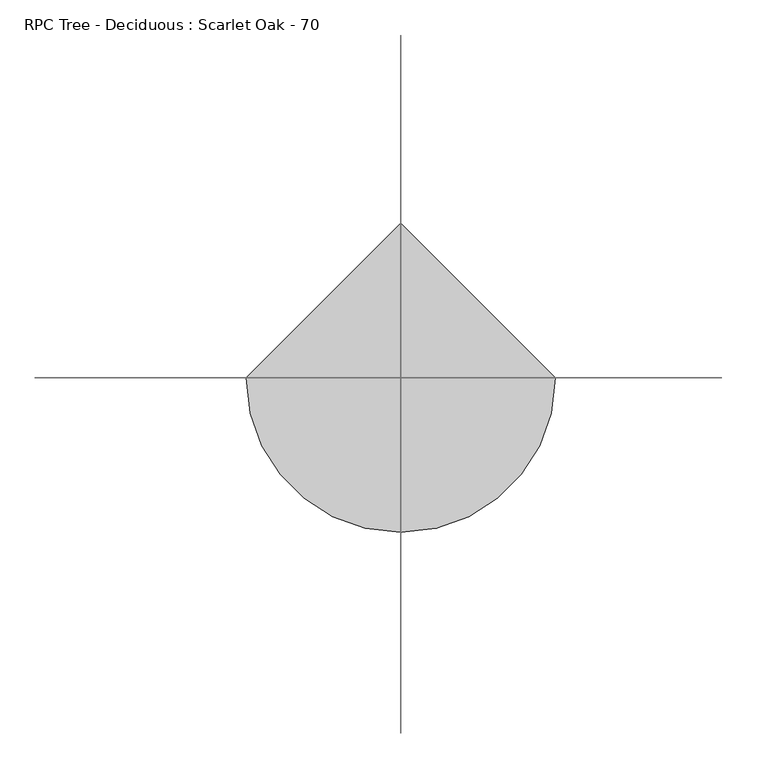
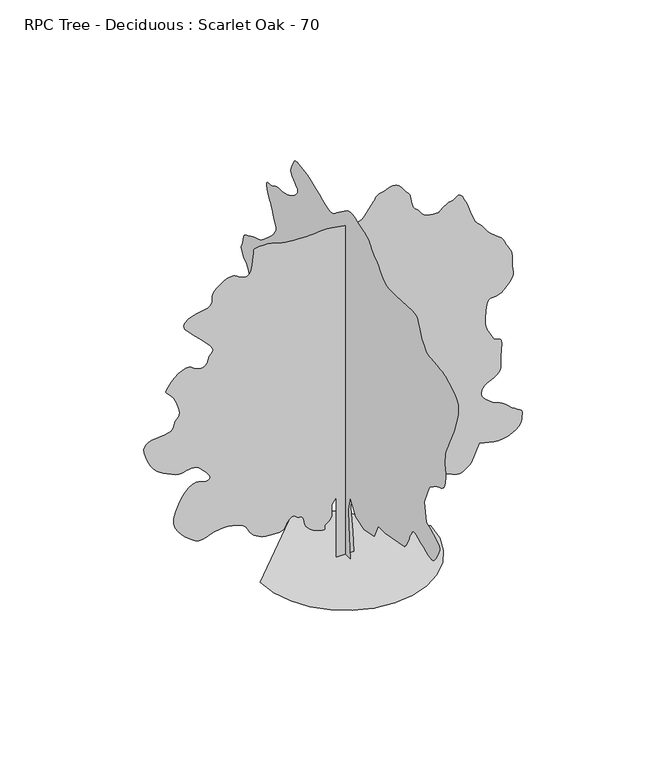
"""IFC4 building model written with IfcOpenShell, lengths in millimetres: geographic element geometry, RPC Tree - Deciduous : Scarlet Oak - 70."""

from ifc_helpers import new_model, si_unit, origin, place, context, project, spatial, triangles, source, transform, mapped, element, save


def rpc_tree_deciduous_scarlet_oak_70_be676745(model_context):
    return source(origin(), model_context, "Body", "Tessellation", [
        triangles([(0.0294444, 522.318082, 0.0), (0.0294444, -501.0802431, 0.0), (0.0294444, -336.0164085, 1947.7549484), (0.0294444, -303.0027805, 2872.1116081), (0.0294444, -501.0802431, 3730.4458443), (0.0294444, -1029.2870281, 2872.1116081), (0.0294444, -1887.6171947, 2608.0102867), (0.0294444, -2878.0002022, 2839.1005417), (0.0294444, -3274.1542191, 3664.4196419), (0.0294444, -3967.424984, 3664.4196419), (0.0294444, -5882.1647964, 4027.5625923), (0.0294444, -5952.6157288, 4112.5481026), (0.0294444, -6021.3603699, 4198.1097404), (0.0294444, -6086.605806, 4284.8236336), (0.0294444, -6146.6457458, 4373.2824783), (0.0294444, -6199.7721542, 4464.0458336), (0.0294444, -6244.2363007, 4557.7110466), (0.0294444, -6278.3313126, 4654.7897141), (0.0294444, -6311.444989, 4754.8129692), (0.0294444, -6353.2209274, 4856.5430969), (0.0294444, -6402.2080536, 4959.7240082), (0.0294444, -6456.956456, 5064.0571747), (0.0294444, -6516.0569183, 5169.2431961), (0.0294444, -6578.0170898, 5275.0274368), (0.0294444, -6641.4701935, 5381.0674759), (0.0294444, -6671.6817215, 5415.3328262), (0.0294444, -6713.4576599, 5442.9840454), (0.0294444, -6778.3193985, 5457.3221237), (0.0294444, -6877.8301849, 5451.7317673), (0.0294444, -7023.555011, 5419.6000076), (0.0294444, -7227.0152664, 5354.2266724), (0.0294444, -7499.7747803, 5249.0400696), (0.0294444, -7787.768248, 5125.2487885), (0.0294444, -8033.0038605, 5014.7706482), (0.0294444, -8241.2859146, 4926.7812515), (0.0294444, -8418.3751053, 4870.5820656), (0.0294444, -8570.0739853, 4855.3908417), (0.0294444, -8702.1008102, 4890.4247498), (0.0294444, -8820.3023163, 4984.9428177), (0.0294444, -8939.5706177, 5133.8255905), (0.0294444, -9062.8503021, 5315.0534821), (0.0294444, -9178.0641998, 5512.4542236), (0.0294444, -9273.0525879, 5709.8549652), (0.0294444, -9335.6946945, 5891.0828568), (0.0294444, -9353.9156754, 6040.0080688), (0.0294444, -9315.5110428, 6140.3728729), (0.0294444, -9221.6754913, 6215.9450043), (0.0294444, -9086.2343399, 6300.1369583), (0.0294444, -8916.1865799, 6391.5831207), (0.0294444, -8718.3591202, 6488.7893967), (0.0294444, -8499.7928101, 6590.3488953), (0.0294444, -8267.3587418, 6694.7675217), (0.0294444, -8028.011142, 6800.6366409), (0.0294444, -7829.9278839, 7923.0809189), (0.0294444, -8325.0935898, 9078.5103928), (0.0294444, -8340.7118225, 9100.5718369), (0.0294444, -8364.9492966, 9127.4981003), (0.0294444, -8406.5548965, 9164.2813202), (0.0294444, -8474.1042618, 9215.7863159), (0.0294444, -8576.3038376, 9286.8779068), (0.0294444, -8721.8583252, 9382.5488113), (0.0294444, -8919.3439453, 9507.7057068), (0.0294444, -9133.6000534, 9621.0854141), (0.0294444, -9323.5762482, 9695.164032), (0.0294444, -9489.3138062, 9755.4161682), (0.0294444, -9630.8144714, 9827.2338776), (0.0294444, -9748.034642, 9936.0039825), (0.0294444, -9841.0167572, 10107.1191193), (0.0294444, -9909.7183777, 10366.0102936), (0.0294444, -9949.4892059, 10620.2924469), (0.0294444, -9960.9245544, 10783.3429596), (0.0294444, -9952.1774139, 10889.2120789), (0.0294444, -9931.2682251, 10971.9953979), (0.0294444, -9906.3476532, 11065.7454895), (0.0294444, -9885.4803223, 11204.5149261), (0.0294444, -9876.7331818, 11422.4411591), (0.0294444, -9879.8050873, 11662.8555542), (0.0294444, -9893.2903107, 11862.2608246), (0.0294444, -9923.5012573, 12044.3857544), (0.0294444, -9976.7991669, 12232.825415), (0.0294444, -10059.582486, 12451.3051025), (0.0294444, -10178.1682709, 12723.5105804), (0.0294444, -10338.8712524, 13073.0787781), (0.0294444, -10491.4654266, 13389.0653046), (0.0294444, -10593.1964264, 13579.7234344), (0.0294444, -10661.9829254, 13697.6267029), (0.0294444, -10715.7924316, 13795.303299), (0.0294444, -10772.5040863, 13925.3244324), (0.0294444, -10849.9528473, 14140.2636383), (0.0294444, -10966.1492432, 14492.6060852), (0.0294444, -11091.3485779, 14900.2091125), (0.0294444, -11175.5829712, 15251.2283844), (0.0294444, -11206.0938995, 15553.7308502), (0.0294444, -11170.1635345, 15815.8218292), (0.0294444, -11055.1635773, 16045.5682709), (0.0294444, -10848.332016, 16251.0336365), (0.0294444, -10536.9545105, 16440.369754), (0.0294444, -10234.8369049, 16595.9939758), (0.0294444, -10036.1129883, 16703.1432495), (0.0294444, -9898.5806854, 16773.8505615), (0.0294444, -9780.0809418, 16820.3640015), (0.0294444, -9638.4953979, 16854.7142303), (0.0294444, -9431.664418, 16889.0656219), (0.0294444, -9117.4277847, 16935.5778992), (0.0294444, -8780.3611496, 16972.2338013), (0.0294444, -8518.9526871, 16986.4003784), (0.0294444, -8311.8228882, 17003.9807007), (0.0294444, -8137.6358459, 17051.0487579), (0.0294444, -7974.9701935, 17153.5471527), (0.0294444, -7802.4900238, 17337.5056915), (0.0294444, -7598.8164093, 17628.8274445), (0.0294444, -7420.9592422, 17949.1230103), (0.0294444, -7315.8580994, 18206.5212524), (0.0294444, -7247.1564789, 18406.6950806), (0.0294444, -7178.4118378, 18555.4929749), (0.0294444, -7073.3106949, 18658.6738861), (0.0294444, -6895.4541092, 18721.9990906), (0.0294444, -6608.4419769, 18751.2717224), (0.0294444, -5023.817189, 18652.2300934), (0.0294444, -4731.7274597, 18657.3507111), (0.0294444, -4493.916394, 18656.6681946), (0.0294444, -4291.8644829, 18668.701181), (0.0294444, -4107.1713959, 18711.8857544), (0.0294444, -3921.3179146, 18804.7824097), (0.0294444, -3715.830748, 18965.7842102), (0.0294444, -3472.2290474, 19213.451651), (0.0294444, -3237.4861084, 19463.5956848), (0.0294444, -3061.6392838, 19634.0271423), (0.0294444, -2930.8408722, 19746.1691345), (0.0294444, -2831.2231155, 19821.3575684), (0.0294444, -2748.9345337, 19880.9283508), (0.0294444, -2670.1064964, 19946.2592468), (0.0294444, -2580.8878143, 20038.7722046), (0.0294444, -2495.2282173, 20148.0120483), (0.0294444, -2425.156477, 20249.7407227), (0.0294444, -2353.9368416, 20344.5581909), (0.0294444, -2264.8121944, 20432.9760498), (0.0294444, -2141.0377728, 20515.6733276), (0.0294444, -1965.8648895, 20593.166272), (0.0294444, -1722.5534328, 20666.006012), (0.0294444, -1449.4057159, 20746.2732056), (0.0294444, -1194.7349236, 20835.2003357), (0.0294444, -956.808676, 20917.2162598), (0.0294444, -733.9029505, 20976.701001), (0.0294444, -524.2767197, 20998.0810913), (0.0294444, -326.1984395, 20965.7342285), (0.0294444, -137.9389459, 20864.08927), (0.0294444, 852.4457148, 20137.8126709), (0.0294444, 959.6634436, 20040.2209534), (0.0294444, 1063.4204098, 19951.2938232), (0.0294444, 1176.4115507, 19879.6470337), (0.0294444, 1311.3532413, 19834.0312134), (0.0294444, 1480.9402737, 19823.0644409), (0.0294444, 1697.8805202, 19855.4089783), (0.0294444, 1974.8814903, 19939.7294128), (0.0294444, 2289.2248032, 20064.9287476), (0.0294444, 2605.876696, 20205.7457336), (0.0294444, 2919.0633934, 20349.4671936), (0.0294444, 3223.0119919, 20483.3287903), (0.0294444, 3511.9481346, 20594.701062), (0.0294444, 3780.0904884, 20670.8289734), (0.0294444, 4021.6737076, 20699.0342285), (0.0294444, 4241.4047722, 20714.4402649), (0.0294444, 4445.5263245, 20749.4730103), (0.0294444, 4630.6374092, 20787.3660461), (0.0294444, 4793.1751625, 20811.432019), (0.0294444, 4929.7682785, 20804.9045105), (0.0294444, 5036.8751129, 20751.0101257), (0.0294444, 5111.0816299, 20632.9777954), (0.0294444, 5177.3938614, 20484.6938232), (0.0294444, 5253.52061, 20347.9300781), (0.0294444, 5325.0389191, 20218.0798645), (0.0294444, 5377.5252502, 20090.5318359), (0.0294444, 5396.4717682, 19960.7234802), (0.0294444, 5367.497374, 19823.9597351), (0.0294444, 5276.1796921, 19675.6315796), (0.0294444, 5136.42892, 19539.7212708), (0.0294444, 4986.82061, 19433.2556763), (0.0294444, 4849.971405, 19341.2543152), (0.0294444, 4748.3267372, 19248.6564789), (0.0294444, 4704.459938, 19140.4828491), (0.0294444, 4740.8164398, 19001.7134125), (0.0294444, 4880.0125946, 18817.2851349), (0.0294444, 5072.2072586, 18633.5393738), (0.0294444, 5253.4351501, 18499.5068573), (0.0294444, 5424.8485245, 18404.0917511), (0.0294444, 5587.5996368, 18336.4575073), (0.0294444, 5742.8401611, 18285.5071289), (0.0294444, 5891.7659546, 18240.4029053), (0.0294444, 6035.4420685, 18190.0490021), (0.0294444, 6178.9484253, 18151.260672), (0.0294444, 6326.5080231, 18138.4591278), (0.0294444, 6478.0790039, 18137.221994), (0.0294444, 6633.7038071, 18133.0827118), (0.0294444, 6793.3824326, 18111.6189056), (0.0294444, 6957.1148804, 18058.3640167), (0.0294444, 7124.8587112, 17958.9805481), (0.0294444, 7298.2347565, 17870.6917511), (0.0294444, 7468.6667953, 17839.0297302), (0.0294444, 7621.2191116, 17831.6046021), (0.0294444, 7740.8716919, 17816.1148499), (0.0294444, 7812.5603394, 17760.2147736), (0.0294444, 7821.3080612, 17631.5156525), (0.0294444, 7752.136702, 17397.7589905), (0.0294444, 7649.8946869, 17151.7542389), (0.0294444, 7565.0202164, 16986.0166809), (0.0294444, 7490.5148804, 16867.6018158), (0.0294444, 7419.5087494, 16763.6523468), (0.0294444, 7345.0034134, 16641.2260986), (0.0294444, 7260.0859222, 16467.4239166), (0.0294444, 7157.8863464, 16209.3001373), (0.0294444, 7049.8836365, 15955.4016815), (0.0294444, 6956.9439606, 15795.0405396), (0.0294444, 6885.8953903, 15696.4686493), (0.0294444, 6843.735173, 15627.9367859), (0.0294444, 6837.3774216, 15557.6992126), (0.0294444, 6873.7763626, 15453.9206635), (0.0294444, 6959.8030884, 15284.9402802), (0.0294444, 7112.9530426, 15060.953952), (0.0294444, 7327.8492279, 14823.1428864), (0.0294444, 7577.4374817, 14585.886438), (0.0294444, 7834.4938843, 14363.6511658), (0.0294444, 8071.9636917, 14170.8594452), (0.0294444, 8262.6218216, 14021.9766724), (0.0294444, 8379.3728348, 13931.3833649), (0.0294444, 8483.0229034, 13874.7158936), (0.0294444, 8638.6477066, 13817.4496216), (0.0294444, 8825.4659546, 13759.0310944), (0.0294444, 9022.6957764, 13698.8638367), (0.0294444, 9209.513443, 13636.3920685), (0.0294444, 9365.1382462, 13571.0611725), (0.0294444, 9468.7888962, 13502.2316528), (0.0294444, 9555.5835983, 13445.0514221), (0.0294444, 9666.1041779, 13404.641098), (0.0294444, 9787.5490906, 13365.3830292), (0.0294444, 9907.285968, 13311.6584015), (0.0294444, 10012.60047, 13227.9356049), (0.0294444, 10090.7329102, 13098.5539673), (0.0294444, 10129.0526642, 12907.9807159), (0.0294444, 10160.4170288, 12716.555191), (0.0294444, 10214.3114136, 12581.1564789), (0.0294444, 10272.8148193, 12480.9625946), (0.0294444, 10318.0899628, 12395.1922485), (0.0294444, 10332.1286407, 12303.1060089), (0.0294444, 10297.0947327, 12183.8377075), (0.0294444, 10195.0660767, 12016.6490753), (0.0294444, 10068.4156677, 11860.0423553), (0.0294444, 9966.0033142, 11766.420163), (0.0294444, 9879.7632294, 11705.6971252), (0.0294444, 9801.5877686, 11647.8343781), (0.0294444, 9723.4553284, 11562.831427), (0.0294444, 9637.2152435, 11420.6912659), (0.0294444, 9534.8023087, 11191.3296844), (0.0294444, 9423.1724945, 10961.5832428), (0.0294444, 9320.7595596, 10816.7548737), (0.0294444, 9236.8239853, 10724.4546936), (0.0294444, 9180.6245087, 10652.339328), (0.0294444, 9161.3797531, 10568.1479553), (0.0294444, 9188.3060165, 10439.4488342), (0.0294444, 9270.7056381, 10233.9834686), (0.0294444, 9380.1588409, 10009.2297455), (0.0294444, 9483.211853, 9834.7438843), (0.0294444, 9581.6988647, 9696.0599075), (0.0294444, 9677.2412888, 9578.7118378), (0.0294444, 9771.6744781, 9468.3191574), (0.0294444, 9866.6628662, 9350.4164703), (0.0294444, 9963.9546021, 9210.5802383), (0.0294444, 10076.865152, 9072.6648193), (0.0294444, 10208.2513184, 8960.1385483), (0.0294444, 10344.2476685, 8858.0244324), (0.0294444, 10471.0259766, 8751.2588562), (0.0294444, 10574.6766266, 8624.9072662), (0.0294444, 10641.3725555, 8463.8630264), (0.0294444, 10657.247168, 8253.1915833), (0.0294444, 10670.6033295, 8087.7522629), (0.0294444, 10719.8038147, 8033.1747803), (0.0294444, 10775.9178314, 8030.5714508), (0.0294444, 10810.0983032, 8021.0557526), (0.0294444, 10793.4132751, 7945.6969803), (0.0294444, 10697.1028748, 7745.6080307), (0.0294444, 10492.1909637, 7361.8587799), (0.0294444, 10277.935437, 6931.4263321), (0.0294444, 10148.5968201, 6614.8003098), (0.0294444, 10067.7331512, 6388.2118149), (0.0294444, 9999.0315308, 6228.064032), (0.0294444, 9906.0488342, 6110.6305023), (0.0294444, 9752.4297226, 6012.2713898), (0.0294444, 9501.8171127, 5909.3038376), (0.0294444, 9212.4580307, 5825.7519608), (0.0294444, 8957.7915985, 5790.718634), (0.0294444, 8723.906456, 5788.0298447), (0.0294444, 8496.9767029, 5801.5144867), (0.0294444, 8263.0915604, 5814.9561081), (0.0294444, 8008.4251282, 5812.2679001), (0.0294444, 7719.1084854, 5777.233992), (0.0294444, 7430.5609818, 5745.8702087), (0.0294444, 7181.2709656, 5752.6122391), (0.0294444, 6962.022139, 5778.9838852), (0.0294444, 6763.5546021, 5806.5072052), (0.0294444, 6576.6514755, 5816.7054199), (0.0294444, 6392.0522781, 5791.1023315), (0.0294444, 6200.4976913, 5711.2205795), (0.0294444, 6017.1786484, 5626.3030884), (0.0294444, 5865.5652283, 5581.838942), (0.0294444, 5749.198494, 5553.5476456), (0.0294444, 5671.5357925, 5517.1911438), (0.0294444, 5636.0321457, 5448.4465027), (0.0294444, 5646.1454819, 5323.1611267), (0.0294444, 5705.3319855, 5116.970224), (0.0294444, 5800.7889496, 4897.9347565), (0.0294444, 5915.3209122, 4742.9500305), (0.0294444, 6045.7687637, 4641.4335526), (0.0294444, 6188.8908417, 4582.6313278), (0.0294444, 6341.5286179, 4555.8759842), (0.0294444, 6500.5247269, 4550.4568382), (0.0294444, 6662.6782013, 4555.748085), (0.0294444, 7289.956192, 3862.4988304), (0.0294444, 7339.1148193, 3784.4387695), (0.0294444, 7386.2671738, 3704.9410057), (0.0294444, 7429.4087265, 3622.554174), (0.0294444, 7466.4477448, 3535.8318512), (0.0294444, 7495.422139, 3443.3401131), (0.0294444, 7514.283197, 3343.6284668), (0.0294444, 7521.0252274, 3235.2545586), (0.0294444, 7519.8729721, 3122.2591301), (0.0294444, 7511.8083481, 3010.4200264), (0.0294444, 7489.8323639, 2900.8938629), (0.0294444, 7447.1175293, 2794.828244), (0.0294444, 7376.6660156, 2693.3841454), (0.0294444, 7271.5648727, 2597.7135315), (0.0294444, 7124.8587112, 2508.9727272), (0.0294444, 6984.9370193, 2433.6097401), (0.0294444, 6886.5779068, 2374.9954399), (0.0294444, 6802.6423325, 2329.6650673), (0.0294444, 6705.9900925, 2294.1490665), (0.0294444, 6569.5251663, 2264.9870384), (0.0294444, 6366.0649109, 2238.7097179), (0.0294444, 6068.470285, 2211.8561245), (0.0294444, 5729.9537384, 2215.7051628), (0.0294444, 5418.0210342, 2274.9936951), (0.0294444, 5126.8702011, 2376.4421539), (0.0294444, 4850.7396721, 2506.7580368), (0.0294444, 4583.869043, 2652.6706421), (0.0294444, 4320.4118683, 2800.8918274), (0.0294444, 4054.684774, 2938.1378105), (0.0294444, 3817.7230751, 3062.9705978), (0.0294444, 3634.4679817, 3180.8732849), (0.0294444, 3489.9038406, 3288.9614548), (0.0294444, 3369.0184868, 3384.3419701), (0.0294444, 3256.7953949, 3464.1301231), (0.0294444, 3138.2183304, 3525.4412064), (0.0294444, 2998.2754189, 3565.3820824), (0.0294444, 2844.3746384, 3599.0675262), (0.0294444, 2692.7867981, 3640.8391045), (0.0294444, 2541.7747948, 3686.6560753), (0.0294444, 2389.6106815, 3732.4686859), (0.0294444, 2234.5534309, 3774.2402641), (0.0294444, 2074.8790203, 3807.9254173), (0.0294444, 1908.8551426, 3829.4834038), (0.0294444, 1739.0759708, 3840.744635), (0.0294444, 1569.2927296, 3846.8082184), (0.0294444, 1399.5135578, 3848.5406708), (0.0294444, 1229.7345314, 3846.8082184), (0.0294444, 1059.9554323, 3842.4770874), (0.0294444, 890.1720457, 3836.4132133), (0.0294444, 720.3929466, 3829.4834038), (0.0294444, 390.2661495, 3334.2918274), (0.0294444, 324.2397655, 2574.9992203), (478.6859705, 0.0010255, 0.0157241), (-511.6970369, 0.0010255, 0.0157241), (-511.6970369, 0.0008118, 3631.4213654), (-775.8025732, 0.0008118, 3268.2824844), (-775.8025732, 0.0008546, 2872.1284676), (-769.7388445, 0.0008546, 2780.2131477), (-769.7388445, 0.0008546, 2688.5835663), (-781.8662292, 0.0008546, 2597.534182), (-812.1804399, 0.0008973, 2507.3513145), (-866.753635, 0.0008973, 2418.3246265), (-951.6453283, 0.0008973, 2330.7360775), (-1072.9148884, 0.0008973, 2244.884341), (-1167.9112701, 0.0008973, 2155.7595486), (-1194.188736, 0.0008973, 2065.4784313), (-1188.1250072, 0.0008973, 1985.0204063), (-1186.1023836, 0.0008973, 1925.3435257), (-1224.5072342, 0.0008973, 1897.4318573), (-1339.7129929, 0.0008973, 1912.2560978), (-1568.1063194, 0.0008973, 1980.7830196), (-1828.6488464, 0.0008973, 2087.5227253), (-2023.3568745, 0.0008973, 2208.1181259), (-2163.2015362, 0.0008973, 2340.2690712), (-2259.162394, 0.0008973, 2481.6540459), (-2322.2059296, 0.0008546, 2629.9691208), (-2363.303421, 0.0008546, 2782.9057159), (-2393.4297798, 0.0008546, 2938.1549606), (-2401.1278564, 0.0008546, 2980.4044167), (-2412.5809364, 0.0008546, 3021.5019081), (-2431.540099, 0.0008546, 3060.2948891), (-2461.7648529, 0.0008546, 3095.6145355), (-2506.9969757, 0.0008546, 3126.3170219), (-2571.0049873, 0.0008546, 3151.2460236), (-2657.5311012, 0.0008546, 3169.2452156), (-2744.0572151, 0.0008546, 3198.8852669), (-2812.101899, 0.0008546, 3248.7429794), (-2871.4883904, 0.0008118, 3302.6420151), (-2932.027137, 0.0008118, 3344.4135933), (-3003.5413765, 0.0008118, 3357.8895149), (-3095.8406845, 0.0008118, 3326.8969299), (-3218.74888, 0.0008546, 3235.2673485), (-3326.8329803, 0.0008546, 3107.0679062), (-3388.1440636, 0.0008546, 2981.7528809), (-3432.7064598, 0.0008546, 2866.2570236), (-3490.548278, 0.0008546, 2767.5054932), (-3591.7066383, 0.0008546, 2692.4368195), (-3766.2009293, 0.0008546, 2647.9683128), (-4044.0679802, 0.0008546, 2641.0382126), (-4351.0931351, 0.0008546, 2661.4442345), (-4600.3828606, 0.0008546, 2695.1293877), (-4802.8614899, 0.0008546, 2743.2549385), (-4969.5809647, 0.0008546, 2806.9684914), (-5111.4653275, 0.0008546, 2887.4307312), (-5239.4389114, 0.0008546, 2985.7982735), (-5364.5958069, 0.0008546, 3103.2187225), (-5470.7213058, 0.0008546, 3231.9942924), (-5546.8904938, 0.0008118, 3361.3544197), (-5611.4534134, 0.0008118, 3487.8214096), (-5682.9717224, 0.0008118, 3607.9390778), (-5779.8797607, 0.0008118, 3718.2375778), (-5920.6973282, 0.0008118, 3815.2566559), (-6123.8587646, 0.0008118, 3895.5267563), (-6328.1294357, 0.0008118, 3956.5436714), (-6476.3296921, 0.0007691, 3999.6637138), (-6593.3789429, 0.0007691, 4027.191394), (-6704.0698608, 0.0007691, 4041.4352921), (-6833.1951187, 0.0007691, 4044.7080574), (-7005.6758698, 0.0007691, 4039.3188515), (-7246.3030426, 0.0007691, 4027.5753822), (-7510.8694519, 0.0007691, 3985.9020538), (-7746.0347488, 0.0008118, 3908.4224808), (-7962.6808273, 0.0008118, 3824.0128075), (-8171.8157364, 0.0008118, 3761.549469), (-8384.4504318, 0.0008118, 3749.9045403), (-8611.4656448, 0.0008118, 3817.9492241), (-8863.9130264, 0.0007691, 3994.5643158), (-9128.0527176, 0.0007691, 4230.7539688), (-9371.9232971, 0.0007691, 4465.1980888), (-9579.4373749, 0.0007264, 4708.3431313), (-9734.3790802, 0.0007264, 4970.5198608), (-9820.619165, 0.0007264, 5262.1404327), (-9821.9853607, 0.0006837, 5593.6167114), (-9722.2606339, 0.0006837, 5975.3172501), (-9555.3702393, 0.0006409, 6360.304216), (-9369.4054276, 0.0006409, 6690.4573196), (-9169.6152969, 0.0005982, 6959.3763702), (-8961.1629044, 0.0005982, 7160.703035), (-8749.2107254, 0.0005982, 7288.1214203), (-8539.0084396, 0.0005982, 7335.3167953), (-8335.719104, 0.0005982, 7295.8453674), (-8143.9935974, 0.0005982, 7229.4476761), (-7974.2446564, 0.0005982, 7201.1133591), (-7840.2545792, 0.0005982, 7212.6771881), (-7755.934726, 0.0005982, 7265.8041779), (-7735.1534363, 0.0005982, 7362.2430588), (-7791.7366104, 0.0005982, 7503.7431427), (-7939.5525879, 0.0005555, 7692.0118835), (-8111.9472977, 0.0005555, 7880.8358231), (-8243.3340454, 0.0005555, 8026.34729), (-8349.2886246, 0.0005555, 8133.7523621), (-8445.4286865, 0.0005555, 8208.2576981), (-8547.372464, 0.0005555, 8255.026355), (-8670.6515671, 0.0005127, 8279.3068497), (-8830.9278305, 0.0005127, 8286.2197998), (-8995.3003555, 0.0005555, 8270.7294662), (-9131.4240234, 0.0005555, 8235.0130417), (-9255.3862244, 0.0005555, 8195.2858154), (-9383.4022476, 0.0005555, 8167.6340149), (-9531.6019226, 0.0005555, 8168.3171127), (-9716.20112, 0.0005555, 8213.4637756), (-9953.3715271, 0.0005127, 8319.2480164), (-10205.0515137, 0.0005127, 8445.8129654), (-10426.6903107, 0.0005127, 8555.6080078), (-10624.6875275, 0.0005127, 8668.3476379), (-10805.3183624, 0.0005127, 8803.5748489), (-10975.0254456, 0.0005127, 8980.919838), (-11140.0804871, 0.00047, 9220.0965179), (-11306.8854218, 0.00047, 9540.7339233), (-11444.8014221, 0.0004273, 9873.4473358), (-11520.9281708, 0.0004273, 10140.9158936), (-11538.1678162, 0.0004273, 10350.6484406), (-11499.3783234, 0.0003846, 10510.1131256), (-11407.4630035, 0.0003846, 10626.8641388), (-11265.3228424, 0.0003846, 10708.3673035), (-11075.7739471, 0.0003846, 10762.1768097), (-10852.0015594, 0.0003846, 10793.0714355), (-10615.5566895, 0.0003846, 10811.2924164), (-10381.9267639, 0.0003846, 10832.3295044), (-10166.8178009, 0.0003846, 10871.8863922), (-9985.8032684, 0.0003846, 10945.5388733), (-9854.4159393, 0.0003846, 11068.8185577), (-9788.2746277, 0.0003418, 11257.3861176), (-9739.4148193, 0.0003418, 11439.466864), (-9663.9275665, 0.0003418, 11558.0526489), (-9583.8748947, 0.0003418, 11650.6504852), (-9521.1048889, 0.0003418, 11754.770874), (-9497.6348099, 0.0002991, 11908.0057068), (-9535.356926, 0.0002991, 12147.8654846), (-9656.24664, 0.0002991, 12511.8572205), (-9827.4466553, 0.0002564, 12870.3876617), (-9991.1796844, 0.0002564, 13096.0796997), (-10131.7838928, 0.0002564, 13229.984317), (-10233.7265076, 0.0002136, 13313.0234344), (-10281.3491821, 0.0002136, 13386.2491974), (-10259.1168182, 0.0002136, 13490.7102631), (-10151.4129272, 0.0002136, 13667.329715), (-9977.8235229, 0.0002136, 13887.7302155), (-9777.0508942, 0.0001709, 14088.5016815), (-9562.4110886, 0.0001709, 14258.0808655), (-9347.173645, 0.0001709, 14384.9440521), (-9144.694725, 0.0001709, 14457.4872986), (-8968.160733, 0.0001709, 14464.2287476), (-8830.9278305, 0.0001709, 14393.6074768), (-8696.383136, 0.0001709, 14288.2929749), (-8530.6449966, 0.0001709, 14206.106131), (-8351.0385178, 0.0001709, 14157.9718597), (-8174.8882233, 0.0001709, 14154.8999542), (-8019.5622391, 0.0001709, 14207.8560242), (-7902.3420685, 0.0001709, 14327.7638214), (-7840.5533981, 0.0001709, 14525.6343018), (-7783.9277847, 0.0001709, 14714.2867401), (-7694.9989105, 0.0001282, 14826.1299133), (-7610.12444, 0.0001282, 14901.5741455), (-7565.6602936, 0.0001282, 14981.0727814), (-7598.0054123, 0.0001282, 15105.0349823), (-7743.5168793, 0.0001282, 15313.914093), (-8038.6366562, 8.55e-05, 15648.0785797), (-8408.6884872, 8.55e-05, 16025.5543762), (-8739.4816681, 4.27e-05, 16343.5465942), (-9007.9309799, 4.27e-05, 16611.3139709), (-9190.8663254, 4.27e-05, 16838.0722229), (-9265.2862015, 0.0, 17033.0835754), (-9208.0199295, 0.0, 17205.5637451), (-8995.982872, 0.0, 17364.7307739), (-8713.1954819, 0.0, 17487.3697998), (-8459.894664, 0.0, 17557.437616), (-8237.189653, 0.0, 17595.1585693), (-8046.2321228, -4.27e-05, 17620.7628204), (-7888.1754913, -4.27e-05, 17654.4305328), (-7764.2132904, -4.27e-05, 17716.4325623), (-7675.455336, -4.27e-05, 17826.9107025), (-7631.2045486, -4.27e-05, 17957.6155151), (-7624.4625183, -4.27e-05, 18072.1468964), (-7632.1434448, -4.27e-05, 18178.6136536), (-7631.2045486, -4.27e-05, 18285.0804108), (-7598.4751511, -8.55e-05, 18399.611792), (-7510.8694519, -8.55e-05, 18530.3154419), (-7345.3446716, -8.55e-05, 18685.2583099), (-7142.7378525, -8.55e-05, 18838.5780212), (-6957.4561386, -8.55e-05, 18957.8463226), (-6786.6404022, -0.0001282, 19041.2703003), (-6627.3454742, -0.0001282, 19087.1861023), (-6476.7133896, -0.0001282, 19093.8426727), (-6331.8419998, -0.0001282, 19059.4482605), (-6189.9151978, -8.55e-05, 18982.383197), (-6043.5927338, -8.55e-05, 18888.1633667), (-5892.7042694, -8.55e-05, 18814.724826), (-5744.6755142, -8.55e-05, 18778.7956238), (-5607.0153122, -8.55e-05, 18797.1863617), (-5487.2778534, -8.55e-05, 18886.5843933), (-5392.9725632, -0.0001282, 19063.8014832), (-5331.5675903, -0.0001282, 19345.5214966), (-5294.9122696, -0.0001282, 19648.0239624), (-5268.6266647, -0.0001709, 19881.7817871), (-5251.0027405, -0.0001709, 20054.9433105), (-5240.334787, -0.0001709, 20175.5359497), (-5234.8304718, -0.0001709, 20251.6615356), (-5232.8247803, -0.0001709, 20291.4312012), (-5232.5259613, -0.0001709, 20302.8677124), (-5189.1286102, -0.0001709, 20309.6114868), (-5071.2259232, -0.0001709, 20324.4594177), (-4897.2946793, -0.0001709, 20339.2678162), (-4685.854969, -0.0001709, 20346.0092651), (-4455.3408417, -0.0001709, 20336.5796082), (-4224.242157, -0.0001709, 20302.8677124), (-4011.0569138, -0.0001709, 20236.8554626), (-3815.5766945, -0.0001709, 20163.4157593), (-3619.5200569, -0.0001709, 20110.2050537), (-3414.2250298, -0.0001709, 20073.1212708), (-3191.0249908, -0.0001709, 20048.2018616), (-2941.2658173, -0.0001709, 20031.3889343), (-2656.2765266, -0.0001709, 20018.5873901), (-2327.3992172, -0.0001709, 20005.7858459), (-2009.9792027, -0.0001709, 20003.9510742), (-1748.5705948, -0.0001709, 20019.4408264), (-1518.346566, -0.0001709, 20041.2883301), (-1294.4765099, -0.0001709, 20058.5291382), (-1052.1293839, -0.0001709, 20060.1499695), (-766.4659338, -0.0001709, 20035.2305603), (-412.6608582, -0.0001709, 19972.7576294), (-55.0054861, -0.0001709, 19898.4668152), (233.3518357, -0.0001709, 19847.258313), (463.9598708, -0.0001709, 19822.0412476), (648.37118, -0.0001709, 19825.6666077), (798.1328236, -0.0001709, 19861.1272339), (924.7918802, -0.0001709, 19931.19505), (1039.9038219, -0.0001709, 20038.7722046), (1535.0953983, -0.0002136, 20666.006012), (1609.4000198, -0.0002136, 20762.7442932), (1668.6885521, -0.0002136, 20853.7201355), (1722.1992393, -0.0002136, 20937.1452759), (1779.1791916, -0.0002136, 21011.3523743), (1848.8625835, -0.0002136, 21074.5903748), (1940.492165, -0.0002136, 21125.1151978), (2063.3021107, -0.0002136, 21161.2153198), (2213.831876, -0.0002564, 21202.6081421), (2378.2215511, -0.0002564, 21257.8675598), (2550.1170181, -0.0002564, 21308.4760986), (2723.1733154, -0.0002564, 21336.0), (2891.0278954, -0.0002564, 21321.961322), (3047.3311455, -0.0002564, 21247.8402649), (3185.7378136, -0.0002136, 21095.2007446), (3308.6419395, -0.0002136, 20921.0997437), (3421.15513, -0.0002136, 20785.6591736), (3520.9647354, -0.0002136, 20675.0542969), (3605.7583969, -0.0002136, 20575.4580505), (3673.2269531, -0.0002136, 20472.9596558), (3721.0624054, -0.0001709, 20353.6901917), (3746.9515228, -0.0001709, 20203.8272461), (3764.9504242, -0.0001709, 20048.4995178), (3789.8794258, -0.0001709, 19919.1609009), (3820.5819122, -0.0001709, 19811.4581726), (3855.9015587, -0.0001282, 19721.0776428), (3894.6904701, -0.0001282, 19643.6707397), (3935.7879616, -0.0001282, 19574.970282), (3978.0417778, -0.0001282, 19510.5765381), (4020.7734718, -0.0001282, 19481.6027252), (4065.2419785, -0.0001282, 19448.5745087), (4113.1710297, -0.0001282, 19407.4816681), (4166.3020889, -0.0001282, 19354.2697998), (4226.3585976, -0.0001282, 19284.8845001), (4295.0648689, -0.0001282, 19195.2736908), (4374.1786446, -0.0001282, 19081.424826), (4491.4412544, -8.55e-05, 18973.2081757), (4657.1793938, -8.55e-05, 18899.1301392), (4847.1550072, -8.55e-05, 18852.7027405), (5037.1309113, -8.55e-05, 18827.69729), (5202.8690506, -8.55e-05, 18817.6688324), (5320.1316605, -8.55e-05, 18816.3468201), (5364.5958069, -8.55e-05, 18817.3281555), (5387.3827881, -8.55e-05, 18841.0964722), (5450.0679153, -8.55e-05, 18902.3729645), (5543.9034668, -8.55e-05, 18986.2236603), (5660.2702011, -0.0001282, 19077.5413422), (5790.4622543, -0.0001282, 19161.392038), (5925.9034058, -0.0001282, 19222.7115509), (6057.8453522, -0.0001282, 19246.4798676), (6176.1317368, -0.0001282, 19275.4548431), (6280.5503632, -0.0001282, 19340.7857391), (6377.5008408, -0.0001282, 19410.1698761), (6473.2572052, -0.0001282, 19451.3057373), (6574.2190659, -0.0001282, 19431.7615814), (6686.7453369, -0.0001282, 19319.2358917), (6817.1507492, -0.0001282, 19081.424826), (6939.9606949, -8.55e-05, 18802.0081604), (7031.5777771, -8.55e-05, 18576.3161224), (7101.260733, -8.55e-05, 18389.2845154), (7158.228186, -4.27e-05, 18225.9793671), (7211.7388733, -4.27e-05, 18071.2934601), (7271.0526947, -4.27e-05, 17910.2916595), (7345.3446716, -4.27e-05, 17727.8690735), (7421.6847794, 0.0, 17567.8067505), (7487.0156754, 0.0, 17466.0757507), (7550.6396988, 0.0, 17396.1369965), (7621.7737289, 0.0, 17331.3607178), (7709.6358078, 0.0, 17245.2055115), (7823.4846725, 0.0, 17111.1311371), (7972.5802231, 0.0, 16902.5496826), (8156.1126251, 4.27e-05, 16670.4138519), (8357.567189, 4.27e-05, 16476.3849976), (8562.4779373, 4.27e-05, 16310.0486389), (8756.4224945, 8.55e-05, 16161.0809875), (8924.9343018, 8.55e-05, 16019.025705), (9053.6328415, 8.55e-05, 15873.4717987), (9128.0527176, 8.55e-05, 15714.0919922), (9186.4706635, 8.55e-05, 15557.7840912), (9267.9744095, 0.0001282, 15417.6496216), (9359.335112, 0.0001282, 15277.515152), (9447.1966095, 0.0001282, 15121.207251), (9518.331221, 0.0001282, 14932.5966705), (9559.4240616, 0.0001709, 14695.4262634), (9557.205011, 0.0001709, 14393.6074768), (9552.6820313, 0.0001709, 14103.5228577), (9577.6026031, 0.0002136, 13891.9543762), (9604.8271042, 0.0002136, 13728.3504089), (9607.2595139, 0.0002136, 13582.0279449), (9557.6747498, 0.0002136, 13422.4772186), (9429.0186493, 0.0002564, 13218.9745239), (9194.0667114, 0.0002564, 12941.0089325), (8915.2476837, 0.0002564, 12707.635968), (8673.3827957, 0.0002564, 12613.970755), (8469.0266647, 0.0002564, 12593.6592041), (8302.8187866, 0.0002564, 12580.3030426), (8175.2725021, 0.0002991, 12507.4191193), (8087.0267258, 0.0002991, 12308.6952026), (8038.5942169, 0.0002991, 11917.6493042), (8020.5011353, 0.0003418, 11484.9129272), (8023.2323639, 0.0003418, 11180.362912), (8047.2564789, 0.0003846, 10966.5329407), (8093.2995987, 0.0003846, 10805.7881012), (8161.8308807, 0.0003846, 10660.6609131), (8253.4473816, 0.0003846, 10493.5571594), (8368.7473206, 0.0004273, 10267.0116852), (8500.3049881, 0.0004273, 10069.9946411), (8633.0579315, 0.0004273, 9980.3838318), (8755.9527557, 0.0004273, 9943.8988495), (8858.0668716, 0.0004273, 9906.2616119), (8928.4335068, 0.0004273, 9813.1940369), (8956.0422867, 0.00047, 9610.37444), (8929.9694595, 0.00047, 9243.6084549), (8894.5518539, 0.0005127, 8839.2488342), (8889.1324173, 0.0005127, 8543.4889801), (8895.3198303, 0.0005127, 8331.4519226), (8894.5518539, 0.0005555, 8178.344989), (8868.3511276, 0.0005555, 8059.2900467), (8798.2838928, 0.0005555, 7949.4519836), (8665.8722076, 0.0005555, 7824.0392899), (8505.8953445, 0.0005555, 7706.4354218), (8364.3946793, 0.0005555, 7626.9373672), (8239.664502, 0.0005555, 7571.1221695), (8129.9549194, 0.0005982, 7524.5244324), (8033.5160385, 0.0005982, 7472.7630569), (7948.641568, 0.0005982, 7401.3302078), (7873.5385941, 0.0005982, 7295.8453674), (7813.8835144, 0.0005982, 7173.7179382), (7780.1722, 0.0005982, 7058.5034592), (7778.2519684, 0.0005982, 6945.0388733), (7813.8835144, 0.0006409, 6828.074501), (7892.783931, 0.0006409, 6702.4908875), (8020.7999542, 0.0006409, 6562.9964951), (8203.6922791, 0.0006409, 6404.5125641), (8397.5083557, 0.0006409, 6265.6152283), (8561.92332, 0.0006409, 6174.6382233), (8707.8190659, 0.0006837, 6110.8438614), (8846.2472443, 0.0006837, 6053.407251), (8988.0885864, 0.0006837, 5981.5046631), (9144.3964874, 0.0006837, 5874.3553894), (9326.0935364, 0.0006837, 5711.2205795), (9519.0137375, 0.0006837, 5542.7087723), (9696.8709045, 0.0006837, 5422.1178772), (9852.7939453, 0.0007264, 5332.6774063), (9979.8292145, 0.0007264, 5257.7023315), (10071.0608551, 0.0007264, 5180.4233276), (10119.5799866, 0.0007264, 5084.0699066), (10118.4277313, 0.0007264, 4951.9151825), (10099.4812134, 0.0007264, 4801.8801544), (10088.0016815, 0.0007691, 4661.062587), (10067.3064331, 0.0007691, 4526.6030617), (10020.6232361, 0.0007691, 4395.6427414), (9931.2252045, 0.0007691, 4265.2114586), (9782.3424316, 0.0007691, 4132.4843857), (9557.205011, 0.0007691, 3994.5643158), (9288.3714203, 0.0008118, 3882.9173515), (9019.5808502, 0.0008118, 3824.9772835), (8750.7472595, 0.0008118, 3811.7917511), (8481.9136688, 0.0008118, 3834.4078125), (8213.1225174, 0.0008118, 3883.8774673), (7944.2889267, 0.0008118, 3951.2521339), (7675.455336, 0.0007691, 4027.5753822), (7213.274826, 0.0008546, 3004.1814537), (7100.0235992, 0.0008546, 2906.0057602), (6986.1317139, 0.0008546, 2813.0320747), (6871.1305939, 0.0008546, 2730.4533943), (6754.380162, 0.0008546, 2663.4624252), (6635.3252197, 0.0008546, 2617.2658264), (6513.3687103, 0.0008546, 2597.0563042), (6387.9560165, 0.0008546, 2608.0274368), (6285.7564407, 0.0008546, 2632.9520782), (6221.0656219, 0.0008546, 2653.8400475), (6174.894603, 0.0008546, 2674.7280167), (6128.125946, 0.0008546, 2699.6526581), (6061.6858154, 0.0008546, 2732.6680847), (5956.5846725, 0.0008546, 2777.8063179), (5793.7481003, 0.0008546, 2839.1174011), (5581.6255829, 0.0008546, 2928.1442345), (5349.8740311, 0.0008546, 3046.0469215), (5111.1670898, 0.0008546, 3181.2744232), (4878.2632828, 0.0008118, 3322.2754097), (4663.7935249, 0.0008118, 3457.5032021), (4480.5599419, 0.0008118, 3575.4058891), (4341.193158, 0.0008118, 3664.436792), (4223.1837914, 0.0008118, 3742.8761902), (4096.524662, 0.0008118, 3835.1757889), (3962.6412643, 0.0008118, 3939.0310776), (3822.9887421, 0.0007691, 4052.1203957), (3679.0007286, 0.0007691, 4172.1395233), (3532.1277168, 0.0007691, 4296.7717415), (3383.8129326, 0.0007691, 4423.7209694), (3350.797506, 0.0007264, 4918.9294052), (2690.5421677, 0.0007264, 4984.9428177), (1502.0799717, 0.0007264, 4885.9011887), (709.7761528, 0.0007691, 4456.7488953), (379.6468122, 0.0008118, 3664.436792), (313.6216999, 0.0008546, 2740.0757721), (412.6591504, 0.00094, 1221.4902672), (-4874.6786179, 0.0, 0.0382848), (-4745.8091583, -1116.9566769, 0.0382848), (-4378.7873749, -2142.7062756, 0.0382848), (-3803.0140892, -3047.8517532, 0.0382848), (-3047.8517532, -3803.0140892, 0.0382848), (-2142.7062756, -4378.7873749, 0.0382848), (-1116.9566769, -4745.8091583, 0.0382848), (0.0002131, -4874.6786179, 0.0382848), (1116.9566769, -4745.8091583, 0.0382848), (2142.7062756, -4378.7873749, 0.0382848), (3047.8517532, -3803.0140892, 0.0382848), (3803.0140892, -3047.8517532, 0.0382848), (4378.7873749, -2142.7062756, 0.0382848), (4745.8091583, -1116.9566769, 0.0382848), (4874.6786179, 0.0004273, 0.0382848), (-0.0006392, 4874.6786179, 0.0382848)], [[1, 2, 3], [368, 1, 3], [368, 3, 4], [367, 368, 4], [367, 4, 5], [277, 278, 279], [366, 367, 5], [276, 277, 279], [276, 279, 280], [7, 8, 9], [6, 7, 9], [5, 6, 9], [315, 316, 317], [201, 202, 203], [200, 201, 203], [200, 203, 204], [199, 200, 204], [199, 204, 205], [198, 199, 205], [198, 205, 206], [198, 206, 207], [197, 198, 207], [197, 207, 208], [275, 276, 280], [196, 197, 208], [195, 196, 208], [194, 195, 208], [194, 208, 209], [193, 194, 209], [192, 193, 209], [192, 209, 210], [191, 192, 210], [191, 210, 211], [191, 211, 212], [190, 191, 212], [190, 212, 213], [190, 213, 214], [189, 190, 214], [189, 214, 215], [188, 189, 215], [187, 188, 215], [186, 187, 215], [10, 11, 12], [314, 315, 317], [10, 12, 13], [10, 13, 14], [10, 14, 15], [10, 15, 16], [10, 16, 17], [10, 17, 18], [10, 18, 19], [10, 19, 20], [10, 20, 21], [10, 21, 22], [185, 186, 215], [185, 215, 216], [275, 280, 281], [10, 22, 23], [167, 168, 169], [166, 167, 169], [165, 166, 169], [165, 169, 170], [164, 165, 170], [164, 170, 171], [163, 164, 171], [163, 171, 172], [163, 172, 173], [163, 173, 174], [163, 174, 175], [163, 175, 176], [163, 176, 177], [163, 177, 178], [163, 178, 179], [163, 179, 180], [162, 163, 180], [161, 162, 180], [160, 161, 180], [159, 160, 180], [159, 180, 181], [158, 159, 181], [157, 158, 181], [156, 157, 181], [156, 181, 182], [155, 156, 182], [154, 155, 182], [154, 182, 183], [9, 10, 23], [9, 23, 24], [9, 24, 25], [45, 46, 47], [44, 45, 47], [44, 47, 48], [43, 44, 48], [43, 48, 49], [42, 43, 49], [42, 49, 50], [41, 42, 50], [40, 41, 50], [40, 50, 51], [39, 40, 51], [38, 39, 51], [37, 38, 51], [36, 37, 51], [35, 36, 51], [34, 35, 51], [33, 34, 51], [33, 51, 52], [32, 33, 52], [32, 52, 53], [31, 32, 53], [30, 31, 53], [29, 30, 53], [28, 29, 53], [28, 53, 54], [27, 28, 54], [26, 27, 54], [5, 9, 25], [5, 25, 26], [5, 26, 54], [5, 54, 55], [366, 5, 55], [365, 366, 55], [364, 365, 55], [363, 364, 55], [362, 363, 55], [361, 362, 55], [361, 55, 56], [153, 154, 183], [153, 183, 184], [313, 314, 317], [360, 361, 56], [184, 185, 216], [153, 184, 216], [152, 153, 216], [152, 216, 217], [243, 244, 245], [242, 243, 245], [242, 245, 246], [241, 242, 246], [241, 246, 247], [241, 247, 248], [240, 241, 248], [240, 248, 249], [240, 249, 250], [239, 240, 250], [239, 250, 251], [238, 239, 251], [237, 238, 251], [236, 237, 251], [235, 236, 251], [234, 235, 251], [233, 234, 251], [232, 233, 251], [231, 232, 251], [230, 231, 251], [229, 230, 251], [228, 229, 251], [228, 251, 252], [227, 228, 252], [226, 227, 252], [226, 252, 253], [226, 253, 254], [226, 254, 255], [226, 255, 256], [226, 256, 257], [225, 226, 257], [224, 225, 257], [223, 224, 257], [222, 223, 257], [222, 257, 258], [221, 222, 258], [220, 221, 258], [115, 116, 117], [114, 115, 117], [114, 117, 118], [113, 114, 118], [113, 118, 119], [112, 113, 119], [111, 112, 119], [110, 111, 119], [152, 217, 218], [313, 317, 318], [313, 318, 319], [313, 319, 320], [313, 320, 321], [313, 321, 322], [313, 322, 323], [313, 323, 324], [313, 324, 325], [313, 325, 326], [313, 326, 327], [313, 327, 328], [313, 328, 329], [313, 329, 330], [313, 330, 331], [313, 331, 332], [313, 332, 333], [313, 333, 334], [313, 334, 335], [313, 335, 336], [313, 336, 337], [313, 337, 338], [313, 338, 339], [313, 339, 340], [313, 340, 341], [312, 313, 341], [312, 341, 342], [312, 342, 343], [311, 312, 343], [311, 343, 344], [311, 344, 345], [310, 311, 345], [310, 345, 346], [310, 346, 347], [310, 347, 348], [309, 310, 348], [309, 348, 349], [309, 349, 350], [308, 309, 350], [308, 350, 351], [307, 308, 351], [307, 351, 352], [307, 352, 353], [307, 353, 354], [307, 354, 355], [307, 355, 356], [307, 356, 357], [307, 357, 358], [306, 307, 358], [306, 358, 359], [306, 359, 360], [306, 360, 56], [305, 306, 56], [305, 56, 57], [304, 305, 57], [303, 304, 57], [302, 303, 57], [301, 302, 57], [301, 57, 58], [301, 58, 59], [110, 119, 120], [109, 110, 120], [109, 120, 121], [301, 59, 60], [300, 301, 60], [300, 60, 61], [151, 152, 218], [109, 121, 122], [300, 61, 62], [145, 146, 147], [144, 145, 147], [143, 144, 147], [143, 147, 148], [142, 143, 148], [141, 142, 148], [140, 141, 148], [140, 148, 149], [139, 140, 149], [138, 139, 149], [137, 138, 149], [136, 137, 149], [135, 136, 149], [134, 135, 149], [133, 134, 149], [132, 133, 149], [132, 149, 150], [131, 132, 150], [130, 131, 150], [129, 130, 150], [128, 129, 150], [127, 128, 150], [126, 127, 150], [126, 150, 151], [126, 151, 218], [125, 126, 218], [124, 125, 218], [123, 124, 218], [123, 218, 219], [122, 123, 219], [109, 122, 219], [108, 109, 219], [108, 219, 220], [108, 220, 258], [108, 258, 259], [108, 259, 260], [108, 260, 261], [108, 261, 262], [107, 108, 262], [107, 262, 263], [107, 263, 264], [106, 107, 264], [106, 264, 265], [106, 265, 266], [106, 266, 267], [106, 267, 268], [105, 106, 268], [104, 105, 268], [103, 104, 268], [102, 103, 268], [101, 102, 268], [100, 101, 268], [99, 100, 268], [98, 99, 268], [97, 98, 268], [96, 97, 268], [95, 96, 268], [94, 95, 268], [93, 94, 268], [92, 93, 268], [91, 92, 268], [90, 91, 268], [89, 90, 268], [88, 89, 268], [87, 88, 268], [86, 87, 268], [85, 86, 268], [84, 85, 268], [83, 84, 268], [82, 83, 268], [81, 82, 268], [80, 81, 268], [79, 80, 268], [78, 79, 268], [77, 78, 268], [76, 77, 268], [75, 76, 268], [74, 75, 268], [73, 74, 268], [72, 73, 268], [71, 72, 268], [70, 71, 268], [69, 70, 268], [68, 69, 268], [67, 68, 268], [66, 67, 268], [65, 66, 268], [64, 65, 268], [63, 64, 268], [62, 63, 268], [300, 62, 268], [299, 300, 268], [298, 299, 268], [297, 298, 268], [296, 297, 268], [295, 296, 268], [294, 295, 268], [293, 294, 268], [292, 293, 268], [291, 292, 268], [290, 291, 268], [289, 290, 268], [288, 289, 268], [287, 288, 268], [286, 287, 268], [285, 286, 268], [284, 285, 268], [283, 284, 268], [282, 283, 268], [281, 282, 268], [275, 281, 268], [275, 268, 269], [274, 275, 269], [274, 269, 270], [274, 270, 271], [273, 274, 271], [272, 273, 271], [802, 369, 370], [802, 370, 371], [801, 802, 371], [800, 801, 371], [575, 576, 577], [799, 800, 371], [574, 575, 577], [383, 384, 385], [383, 385, 386], [382, 383, 386], [382, 386, 387], [381, 382, 387], [381, 387, 388], [794, 795, 796], [510, 511, 512], [574, 577, 578], [573, 574, 578], [572, 573, 578], [572, 578, 579], [571, 572, 579], [571, 579, 580], [570, 571, 580], [570, 580, 581], [570, 581, 582], [569, 570, 582], [569, 582, 583], [569, 583, 584], [568, 569, 584], [568, 584, 585], [509, 510, 512], [509, 512, 513], [508, 509, 513], [508, 513, 514], [508, 514, 515], [507, 508, 515], [507, 515, 516], [507, 516, 517], [507, 517, 518], [507, 518, 519], [507, 519, 520], [507, 520, 521], [507, 521, 522], [506, 507, 522], [506, 522, 523], [505, 506, 523], [505, 523, 524], [504, 505, 524], [568, 585, 586], [504, 524, 525], [538, 539, 540], [538, 540, 541], [537, 538, 541], [537, 541, 542], [536, 537, 542], [536, 542, 543], [536, 543, 544], [535, 536, 544], [535, 544, 545], [535, 545, 546], [534, 535, 546], [534, 546, 547], [533, 534, 547], [533, 547, 548], [381, 388, 389], [380, 381, 389], [380, 389, 390], [380, 390, 391], [380, 391, 392], [380, 392, 393], [379, 380, 393], [378, 379, 393], [377, 378, 393], [376, 377, 393], [375, 376, 393], [374, 375, 393], [373, 374, 393], [372, 373, 393], [372, 393, 394], [372, 394, 395], [372, 395, 396], [372, 396, 397], [372, 397, 398], [371, 372, 398], [371, 398, 399], [532, 533, 548], [371, 399, 400], [567, 568, 586], [567, 586, 587], [657, 658, 659], [657, 659, 660], [656, 657, 660], [656, 660, 661], [655, 656, 661], [655, 661, 662], [654, 655, 662], [654, 662, 663], [653, 654, 663], [652, 653, 663], [651, 652, 663], [650, 651, 663], [649, 650, 663], [649, 663, 664], [648, 649, 664], [647, 648, 664], [647, 664, 665], [647, 665, 666], [647, 666, 667], [647, 667, 668], [647, 668, 669], [793, 794, 796], [713, 714, 715], [713, 715, 716], [712, 713, 716], [712, 716, 717], [711, 712, 717], [646, 647, 669], [711, 717, 718], [567, 587, 588], [645, 646, 669], [645, 669, 670], [750, 751, 752], [749, 750, 752], [748, 749, 752], [748, 752, 753], [747, 748, 753], [747, 753, 754], [747, 754, 755], [747, 755, 756], [747, 756, 757], [747, 757, 758], [747, 758, 759], [747, 759, 760], [746, 747, 760], [746, 760, 761], [746, 761, 762], [745, 746, 762], [745, 762, 763], [745, 763, 764], [744, 745, 764], [743, 744, 764], [743, 764, 765], [742, 743, 765], [741, 742, 765], [741, 765, 766], [740, 741, 766], [739, 740, 766], [738, 739, 766], [737, 738, 766], [736, 737, 766], [735, 736, 766], [644, 645, 670], [567, 588, 589], [792, 793, 796], [371, 400, 401], [371, 401, 402], [371, 402, 403], [371, 403, 404], [371, 404, 405], [799, 371, 405], [799, 405, 406], [766, 767, 768], [488, 489, 490], [488, 490, 491], [487, 488, 491], [487, 491, 492], [486, 487, 492], [486, 492, 493], [485, 486, 493], [485, 493, 494], [485, 494, 495], [484, 485, 495], [483, 484, 495], [483, 495, 496], [482, 483, 496], [481, 482, 496], [480, 481, 496], [479, 480, 496], [479, 496, 497], [478, 479, 497], [477, 478, 497], [476, 477, 497], [475, 476, 497], [474, 475, 497], [473, 474, 497], [472, 473, 497], [471, 472, 497], [471, 497, 498], [470, 471, 498], [469, 470, 498], [469, 498, 499], [468, 469, 499], [468, 499, 500], [468, 500, 501], [468, 501, 502], [468, 502, 503], [467, 468, 503], [466, 467, 503], [466, 503, 504], [466, 504, 525], [465, 466, 525], [465, 525, 526], [464, 465, 526], [463, 464, 526], [735, 766, 768], [735, 768, 769], [735, 769, 770], [735, 770, 771], [735, 771, 772], [735, 772, 773], [735, 773, 774], [735, 774, 775], [735, 775, 776], [735, 776, 777], [735, 777, 778], [735, 778, 779], [735, 779, 780], [735, 780, 781], [735, 781, 782], [735, 782, 783], [735, 783, 784], [735, 784, 785], [735, 785, 786], [735, 786, 787], [735, 787, 788], [735, 788, 789], [735, 789, 790], [735, 790, 791], [735, 791, 792], [735, 792, 796], [734, 735, 796], [733, 734, 796], [732, 733, 796], [731, 732, 796], [731, 796, 797], [730, 731, 797], [567, 589, 590], [455, 456, 457], [454, 455, 457], [453, 454, 457], [453, 457, 458], [452, 453, 458], [451, 452, 458], [451, 458, 459], [450, 451, 459], [449, 450, 459], [448, 449, 459], [447, 448, 459], [446, 447, 459], [445, 446, 459], [444, 445, 459], [443, 444, 459], [442, 443, 459], [441, 442, 459], [440, 441, 459], [439, 440, 459], [438, 439, 459], [437, 438, 459], [437, 459, 460], [436, 437, 460], [435, 436, 460], [434, 435, 460], [434, 460, 461], [433, 434, 461], [432, 433, 461], [431, 432, 461], [430, 431, 461], [429, 430, 461], [428, 429, 461], [428, 461, 462], [427, 428, 462], [411, 412, 413], [411, 413, 414], [410, 411, 414], [410, 414, 415], [409, 410, 415], [409, 415, 416], [409, 416, 417], [408, 409, 417], [408, 417, 418], [408, 418, 419], [408, 419, 420], [408, 420, 421], [408, 421, 422], [408, 422, 423], [408, 423, 424], [408, 424, 425], [408, 425, 426], [407, 408, 426], [407, 426, 427], [407, 427, 462], [406, 407, 462], [799, 406, 462], [799, 462, 463], [799, 463, 526], [798, 799, 526], [798, 526, 527], [798, 527, 528], [798, 528, 529], [798, 529, 530], [798, 530, 531], [797, 798, 531], [730, 797, 531], [729, 730, 531], [728, 729, 531], [728, 531, 532], [728, 532, 548], [728, 548, 549], [728, 549, 550], [727, 728, 550], [726, 727, 550], [725, 726, 550], [724, 725, 550], [723, 724, 550], [722, 723, 550], [721, 722, 550], [720, 721, 550], [719, 720, 550], [718, 719, 550], [711, 718, 550], [710, 711, 550], [709, 710, 550], [708, 709, 550], [707, 708, 550], [706, 707, 550], [705, 706, 550], [704, 705, 550], [703, 704, 550], [702, 703, 550], [701, 702, 550], [701, 550, 551], [701, 551, 552], [701, 552, 553], [701, 553, 554], [701, 554, 555], [701, 555, 556], [701, 556, 557], [701, 557, 558], [701, 558, 559], [700, 701, 559], [699, 700, 559], [698, 699, 559], [697, 698, 559], [696, 697, 559], [617, 618, 619], [616, 617, 619], [615, 616, 619], [615, 619, 620], [614, 615, 620], [613, 614, 620], [613, 620, 621], [612, 613, 621], [612, 621, 622], [611, 612, 622], [610, 611, 622], [609, 610, 622], [608, 609, 622], [607, 608, 622], [606, 607, 622], [605, 606, 622], [604, 605, 622], [604, 622, 623], [604, 623, 624], [604, 624, 625], [604, 625, 626], [604, 626, 627], [604, 627, 628], [604, 628, 629], [604, 629, 630], [604, 630, 631], [604, 631, 632], [603, 604, 632], [603, 632, 633], [602, 603, 633], [602, 633, 634], [602, 634, 635], [602, 635, 636], [602, 636, 637], [602, 637, 638], [602, 638, 639], [602, 639, 640], [602, 640, 641], [601, 602, 641], [643, 644, 670], [643, 670, 671], [567, 590, 591], [566, 567, 591], [692, 693, 694], [692, 694, 695], [691, 692, 695], [691, 695, 696], [690, 691, 696], [680, 681, 682], [689, 690, 696], [679, 680, 682], [679, 682, 683], [678, 679, 683], [559, 560, 561], [559, 561, 562], [559, 562, 563], [566, 591, 592], [642, 643, 671], [642, 671, 672], [642, 672, 673], [642, 673, 674], [642, 674, 675], [642, 675, 676], [600, 601, 641], [688, 689, 696], [687, 688, 696], [686, 687, 696], [685, 686, 696], [684, 685, 696], [683, 684, 696], [678, 683, 696], [677, 678, 696], [676, 677, 696], [642, 676, 696], [641, 642, 696], [600, 641, 696], [599, 600, 696], [598, 599, 696], [597, 598, 696], [596, 597, 696], [595, 596, 696], [594, 595, 696], [593, 594, 696], [592, 593, 696], [566, 592, 696], [565, 566, 696], [564, 565, 696], [564, 696, 559], [564, 559, 563], [817, 818, 803], [816, 817, 803], [816, 803, 804], [815, 816, 804], [815, 804, 805], [815, 805, 806], [814, 815, 806], [813, 814, 806], [813, 806, 807], [813, 807, 808], [813, 808, 809], [813, 809, 810], [813, 810, 811], [813, 811, 812]], closed=False),
    ])


if __name__ == "__main__":
    model = new_model("IFC4")
    model_context = context("Model", 3, world=origin())
    ifc_project = project(units=[si_unit("LENGTHUNIT", "METRE", prefix="MILLI")], contexts=[model_context])
    site = spatial("IfcSite", under=ifc_project)
    building = spatial("IfcBuilding", under=site)
    placement = place(None, origin())
    rpc_tree_deciduous_scarlet_oak_70_shape = rpc_tree_deciduous_scarlet_oak_70_be676745(model_context)
    element("IfcGeographicElement", 1, ObjectType="RPC Tree - Deciduous : Scarlet Oak - 70", at=placement, inside=building, context=model_context, shape_type="MappedRepresentation", body=[
        mapped(rpc_tree_deciduous_scarlet_oak_70_shape, transform((0.0, 0.0, 0.0), x_axis=(1.0, 0.0, 0.0), y_axis=(0.0, 1.0, 0.0), z_axis=(0.0, 0.0, 1.0))),
    ])
    save(model, "model.ifc")

# Revit data of these elements
# Type "RPC Tree - Deciduous : Scarlet Oak - 70"
#   COBie.Type.CreatedBy = "doug.wood@us.ibm.com"
#   COBie.Type.CreatedOn = "2016-04-14T02:07:24"
#   COBie.Type.Name = "Planting_RPC Tree - Deciduous_Scarlet Oak - 70"
#   COBie.Type.Category = "23-40 05 17 24 : Deciduous Trees"
#   COBie.Type.Description = "RPC Tree - Deciduous_Scarlet Oak - 70"
#   COBie.Type.Manufacturer = ""
#   COBie.Type.ModelNumber = ""
#   built-in parameter 1005198 = "{2, 15},{39, RPC-16-G0FB-J5PX-0LX6-U000-ST1L-LVER-AU},{1, 0},{1, 0},{2, 13},{1, 8},{5, Color},{1, 0},{1, 0},{3, 0.8},{3, 0.8},{3, 0.8},{1, 8},{7, BBoxMin},{1, 0},{1, 0},{1, 0},{1, 0},{1, 0},{1, 8},{7, BBoxMax},{1, 0},{1, 0},{1, 0},{1, 0},{1, 0},{2, 11},{9, RPCTypeId},{1, 0},{1, 0},{39, RPC-16-G0FB-J5PX-0LX6-U000-ST1L-LVER-AU},{1, 6},{14, RPCPlantHeight},{1, 0},{1, 0},{2, 42},{2, 11},{7, keyword},{1, 0},{1, 0},{34, :RPCs:Trees [General]:Geometry:RPC},{2, 11},{8, category},{1, 0},{1, 0},{15, Trees [General]},{2, 11},{12, LocalizedUID},{1, 0},{1, 0},{11, Scarlet_Oak},{2, 14},{6, Height},{1, 0},{1, 0},{2, 42},{1, 2},{16, Cast Reflections},{1, 0},{1, 0},{1, 0},{1, 2},{12, Cast Shadows},{1, 0},{1, 0},{1, 1},{1, 2},{9, Lock View},{1, 0},{1, 0},{1, 0},{1, 4},{5, ViewC},{1, 0},{1, 0},{1, 0},{21, assetlibrary_base.fbx},{1, 5},"
#   built-in parameter 1005195 = "RPC-16-G0FB-J5PX-0LX6-U000-ST1L-LVER-AU"
#   Type Comments = "Scarlet Oak"
#   Assembly Code = "G2050500"
#   COBie.Type.ReplacementCost = 0
#   Height = 70' - 0"
#   COBie.Type = no
